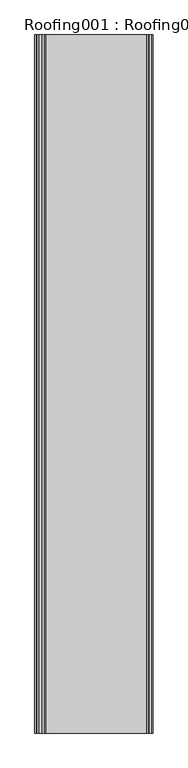
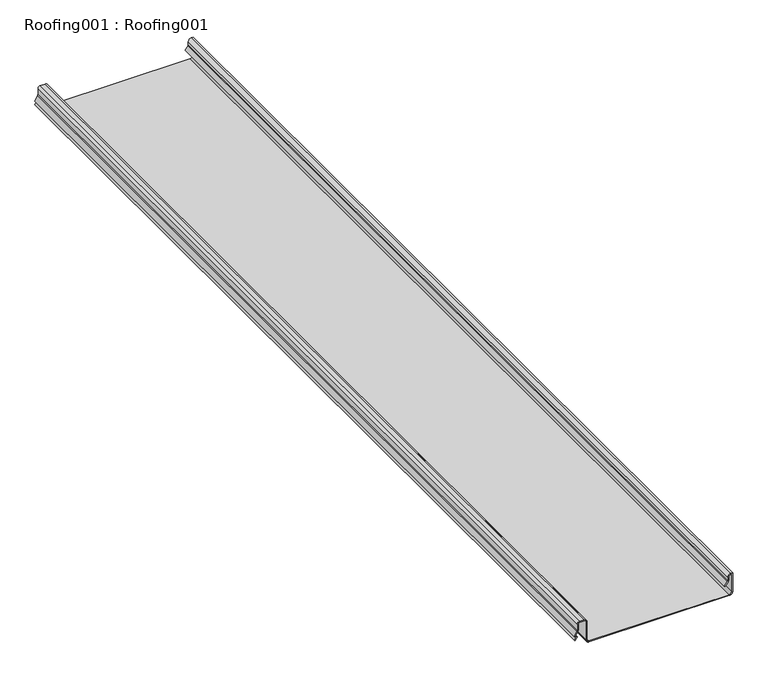
"""IFC4 building model written with IfcOpenShell, lengths in millimetres: proxy geometry, Roofing001 : Roofing001."""

from ifc_helpers import new_model, si_unit, point, frame, frame_2d, origin, place, context, project, spatial, polyline, circle_curve, trimmed, segment, composite_curve, outline, extrude, source, transform, mapped, element, save


def roofing001_roofing001_dc8e391a(model_context):
    return source(origin(), model_context, "Body", "SweptSolid", [
        extrude(outline(composite_curve([segment(trimmed(circle_curve(frame_2d((43490.7540667, -5515.7235547)), 5.08), [point((43487.7710372, -5511.6116287))], [point((43490.7540667, -5510.6435547))], False, "CARTESIAN"), True, "CONTINUOUS"), segment(polyline([(43490.7540667, -5510.6435547), (43497.510625, -5510.6435547)]), True, "CONTINUOUS"), segment(trimmed(circle_curve(frame_2d((43497.510625, -5505.5635547)), 5.08), [point((43497.510625, -5510.6435547))], [point((43502.590625, -5505.5635547))], True, "CARTESIAN"), True, "CONTINUOUS"), segment(polyline([(43502.590625, -5505.5635547), (43502.590625, -5503.96875), (43462.8534375, -5503.96875)]), True, "CONTINUOUS"), segment(trimmed(circle_curve(frame_2d((43462.8534375, -5509.04875)), 5.08), [point((43462.8534375, -5503.96875))], [point((43457.7734375, -5509.04875))], True, "CARTESIAN"), True, "CONTINUOUS"), segment(polyline([(43457.7734375, -5509.04875), (43457.7734375, -5809.322832)]), True, "CONTINUOUS"), segment(trimmed(circle_curve(frame_2d((43462.8534375, -5809.322832)), 5.08), [point((43457.7734375, -5809.322832))], [point((43462.8534375, -5814.402832))], True, "CARTESIAN"), True, "CONTINUOUS"), segment(polyline([(43462.8534375, -5814.402832), (43504.466875, -5814.402832)]), True, "CONTINUOUS"), segment(trimmed(circle_curve(frame_2d((43504.466875, -5819.482832)), 5.08), [point((43504.466875, -5814.402832))], [point((43509.546875, -5819.482832))], False, "CARTESIAN"), True, "CONTINUOUS"), segment(polyline([(43509.546875, -5819.482832), (43509.546875, -5829.4906089)]), True, "CONTINUOUS"), segment(trimmed(circle_curve(frame_2d((43504.466875, -5829.4906089)), 5.08), [point((43509.546875, -5829.4906089))], [point((43504.466875, -5834.5706089))], False, "CARTESIAN"), True, "CONTINUOUS"), segment(polyline([(43504.466875, -5834.5706089), (43491.2843008, -5834.5706089)]), True, "CONTINUOUS"), segment(trimmed(circle_curve(frame_2d((43491.2843008, -5839.6506089)), 5.08), [point((43491.2843008, -5834.5706089))], [point((43488.7802894, -5835.2306172))], True, "CARTESIAN"), True, "CONTINUOUS"), segment(polyline([(43488.7802894, -5835.2306172), (43478.2226563, -5841.2117222), (43475.78125, -5837.0476597), (43470.1796875, -5841.0466832), (43469.0176138, -5839.4189286), (43476.399929, -5834.1486043), (43478.9513272, -5838.5002691), (43487.7944581, -5833.490463)]), True, "CONTINUOUS"), segment(trimmed(circle_curve(frame_2d((43491.2843008, -5839.6506089)), 7.08), [point((43487.7944581, -5833.490463))], [point((43491.2843008, -5832.5706089))], False, "CARTESIAN"), True, "CONTINUOUS"), segment(polyline([(43491.2843008, -5832.5706089), (43504.466875, -5832.5706089)]), True, "CONTINUOUS"), segment(trimmed(circle_curve(frame_2d((43504.466875, -5829.4906089)), 3.08), [point((43504.466875, -5832.5706089))], [point((43507.546875, -5829.4906089))], True, "CARTESIAN"), True, "CONTINUOUS"), segment(polyline([(43507.546875, -5829.4906089), (43507.546875, -5819.482832)]), True, "CONTINUOUS"), segment(trimmed(circle_curve(frame_2d((43504.466875, -5819.482832)), 3.08), [point((43507.546875, -5819.482832))], [point((43504.466875, -5816.402832))], True, "CARTESIAN"), True, "CONTINUOUS"), segment(polyline([(43504.466875, -5816.402832), (43462.8534375, -5816.402832)]), True, "CONTINUOUS"), segment(trimmed(circle_curve(frame_2d((43462.8534375, -5809.322832)), 7.08), [point((43462.8534375, -5816.402832))], [point((43455.7734375, -5809.322832))], False, "CARTESIAN"), True, "CONTINUOUS"), segment(polyline([(43455.7734375, -5809.322832), (43455.7734375, -5509.04875)]), True, "CONTINUOUS"), segment(trimmed(circle_curve(frame_2d((43462.8534375, -5509.04875)), 7.08), [point((43455.7734375, -5509.04875))], [point((43462.8534375, -5501.96875))], False, "CARTESIAN"), True, "CONTINUOUS"), segment(polyline([(43462.8534375, -5501.96875), (43504.590625, -5501.96875), (43504.590625, -5505.5635547)]), True, "CONTINUOUS"), segment(trimmed(circle_curve(frame_2d((43497.510625, -5505.5635547)), 7.08), [point((43504.590625, -5505.5635547))], [point((43497.510625, -5512.6435547))], False, "CARTESIAN"), True, "CONTINUOUS"), segment(polyline([(43497.510625, -5512.6435547), (43490.7540667, -5512.6435547)]), True, "CONTINUOUS"), segment(trimmed(circle_curve(frame_2d((43490.7540667, -5515.7235547)), 3.08), [point((43490.7540667, -5512.6435547))], [point((43488.9454582, -5513.2304972))], True, "CARTESIAN"), True, "CONTINUOUS"), segment(polyline([(43488.9454582, -5513.2304972), (43480.4712961, -5519.3781458), (43479.296875, -5517.7592773), (43487.7710372, -5511.6116287)]), True, "CONTINUOUS")], self_intersect=False)), frame((0.0, 7982.1531721, 0.0), z_axis=(0.0, 1.0, 0.0), x_axis=(0.0, 0.0, 1.0)), (0.0, 0.0, 1.0), 2000.0),
    ])


if __name__ == "__main__":
    model = new_model("IFC4")
    model_context = context("Model", 3, world=origin())
    ifc_project = project(units=[si_unit("LENGTHUNIT", "METRE", prefix="MILLI")], contexts=[model_context])
    site = spatial("IfcSite", under=ifc_project)
    building = spatial("IfcBuilding", under=site)
    placement = place(None, origin())
    roofing001_roofing001_shape = roofing001_roofing001_dc8e391a(model_context)
    element("IfcBuildingElementProxy", 1, Name="Roofing001 : Roofing001", ObjectType="Roofing001 : Roofing001", at=placement, inside=building, context=model_context, shape_type="MappedRepresentation", body=[
        mapped(roofing001_roofing001_shape, transform((0.0, 0.0, 0.0), x_axis=(1.0, 0.0, 0.0), y_axis=(0.0, 1.0, 0.0), z_axis=(0.0, 0.0, 1.0))),
    ])
    save(model, "model.ifc")

# Revit data of these elements
# Type "Roofing001 : Roofing001"
#   NameOverride = "Roofing001"
# Element 1 (IfcBuildingElementProxy, "Roofing001 : Roofing001")
#   Materials on its faces: "STANDING SEAM METAL ROOF"
# Materials
#   "STANDING SEAM METAL ROOF": class "Unassigned", colour RGB 128 128 128, transparency 0
